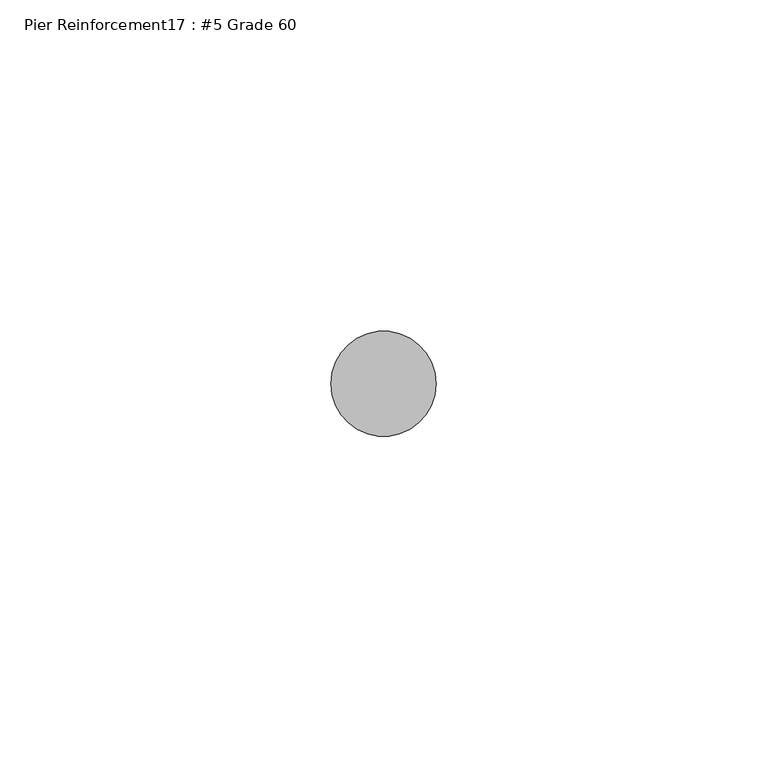
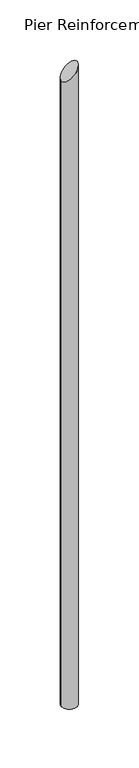
"""IFC4 building model written with IfcOpenShell, lengths in millimetres: proxy geometry, Pier Reinforcement17 : #5 Grade 60."""

from ifc_helpers import new_model, si_unit, frame, origin, place, context, project, spatial, circle_curve, ellipse_curve, source, transform, mapped, element, save
from ifc_brep_helpers import plane_surface, cylinder_surface, advanced_brep


def pier_reinforcement17_5_grade_60_09fa241f(model_context):
    return source(origin(), model_context, "Body", "AdvancedBrep", [
        advanced_brep(
        [(590218.1172365, -534045.8663841, -733.425), (590233.9922365, -534045.8663841, -733.425), (590233.9922365, -534045.8663841, -47.625), (590218.1172365, -534045.8663841, -63.5)],
        [
            (0, 1, circle_curve(frame((590226.0547365, -534045.8663841, -733.425), z_axis=(0.0, 0.0, -1.0), x_axis=(1.0, 0.0, 0.0)), 7.9375)),
            (1, 0, circle_curve(frame((590226.0547365, -534045.8663841, -733.425), z_axis=(0.0, 0.0, -1.0), x_axis=(1.0, 0.0, 0.0)), 7.9375)),
            (1, 2),
            (2, 3, ellipse_curve(frame((590226.0547365, -534045.8663841, -55.5625), z_axis=(0.7071067811865458, 0.0, -0.7071067811865493), x_axis=(0.7071067811865493, 0.0, 0.7071067811865456)), 11.2253202, 7.9375)),
            (3, 0),
            (3, 2, ellipse_curve(frame((590226.0547365, -534045.8663841, -55.5625), z_axis=(0.7071067811865458, 0.0, -0.7071067811865493), x_axis=(0.7071067811865493, 0.0, 0.7071067811865456)), 11.2253202, 7.9375)),
        ],
        [
            plane_surface(frame((590233.9922365, -534045.8663841, -733.425), z_axis=(0.0, 0.0, -1.0), x_axis=(0.0, -1.0, 0.0))),
            cylinder_surface(frame((590226.0547365, -534045.8663841, -733.425), z_axis=(0.0, 0.0, 1.0), x_axis=(1.0, 0.0, 0.0)), 7.9375),
            plane_surface(frame((590233.9922365, -534020.4663841, -47.625), z_axis=(-0.7071067811865458, 0.0, 0.7071067811865493), x_axis=(0.0, -1.0, 0.0))),
        ],
        [
            (0, [[1, 2]]),
            (1, [[-2, 3, 4, 5]]),
            (1, [[-1, -5, 6, -3]]),
            (2, [[-4, -6]]),
        ],
    ),
    ])


if __name__ == "__main__":
    model = new_model("IFC4")
    model_context = context("Model", 3, world=origin())
    ifc_project = project(units=[si_unit("LENGTHUNIT", "METRE", prefix="MILLI")], contexts=[model_context])
    site = spatial("IfcSite", under=ifc_project)
    building = spatial("IfcBuilding", under=site)
    placement = place(None, origin())
    pier_reinforcement17_5_grade_60_shape = pier_reinforcement17_5_grade_60_09fa241f(model_context)
    element("IfcBuildingElementProxy", 1, Name="Pier Reinforcement17 : #5 Grade 60", ObjectType="Pier Reinforcement17 : #5 Grade 60", at=placement, inside=building, context=model_context, shape_type="MappedRepresentation", body=[
        mapped(pier_reinforcement17_5_grade_60_shape, transform((0.0, 0.0, 0.0), x_axis=(1.0, 0.0, 0.0), y_axis=(0.0, 1.0, 0.0), z_axis=(0.0, 0.0, 1.0))),
    ])
    save(model, "model.ifc")

# Revit data of these elements
# Element 1 (IfcBuildingElementProxy, "Pier Reinforcement17 : #5 Grade 60")
#   Materials on its faces: "#5 GR. 60 BEND 24\"x24\""
# Materials
#   "#5 GR. 60 BEND 24\"x24\"": class "Generic", colour RGB 84 83 81, transparency 0, Cost = 0
